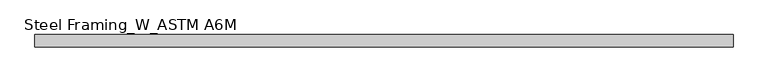
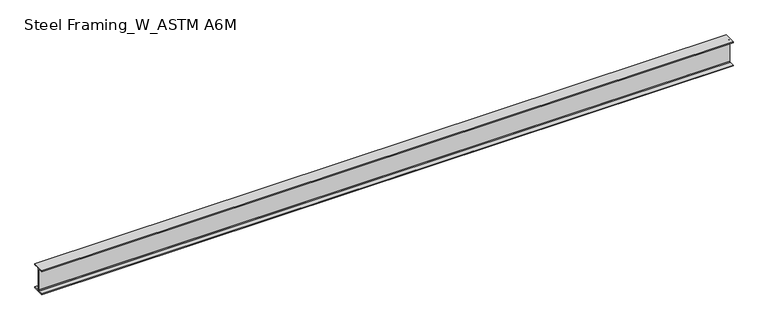
"""IFC4 building model written with IfcOpenShell, lengths in millimetres: beam geometry, Steel Framing_W_ASTM A6M : H_SB_AR_S02_W360x51_B4."""

from ifc_helpers import new_model, si_unit, point, frame, frame_2d, origin, place, context, project, spatial, polyline, circle_curve, trimmed, segment, composite_curve, outline, extrude, source, transform, mapped, element, save


def steel_framing_w_astm_a6m_bf6e2db3(model_context):
    return source(origin(), model_context, "Body", "SweptSolid", [
        extrude(outline(composite_curve([segment(polyline([(85.5, -166.4), (85.5, -178.0), (-85.5, -178.0), (-85.5, -166.4), (-13.72, -166.4)]), True, "CONTINUOUS"), segment(trimmed(circle_curve(frame_2d((-13.72, -156.3)), 10.1), [point((-13.72, -166.4))], [point((-3.62, -156.3))], True, "CARTESIAN"), True, "CONTINUOUS"), segment(polyline([(-3.62, -156.3), (-3.62, 156.3)]), True, "CONTINUOUS"), segment(trimmed(circle_curve(frame_2d((-13.72, 156.3)), 10.1), [point((-3.62, 156.3))], [point((-13.72, 166.4))], True, "CARTESIAN"), True, "CONTINUOUS"), segment(polyline([(-13.72, 166.4), (-85.5, 166.4), (-85.5, 178.0), (85.5, 178.0), (85.5, 166.4), (13.72, 166.4)]), True, "CONTINUOUS"), segment(trimmed(circle_curve(frame_2d((13.72, 156.3)), 10.1), [point((13.72, 166.4))], [point((3.62, 156.3))], True, "CARTESIAN"), True, "CONTINUOUS"), segment(polyline([(3.62, 156.3), (3.62, -156.3)]), True, "CONTINUOUS"), segment(trimmed(circle_curve(frame_2d((13.72, -156.3)), 10.1), [point((3.62, -156.3))], [point((13.72, -166.4))], True, "CARTESIAN"), True, "CONTINUOUS"), segment(polyline([(13.72, -166.4), (85.5, -166.4)]), True, "CONTINUOUS")], self_intersect=False)), frame((-4814.1, 0.0, 0.0), z_axis=(1.0, 0.0, 0.0), x_axis=(0.0, 1.0, 0.0)), (0.0, 0.0, 1.0), 9715.9),
    ])


if __name__ == "__main__":
    model = new_model("IFC4")
    model_context = context("Model", 3, world=origin())
    ifc_project = project(units=[si_unit("LENGTHUNIT", "METRE", prefix="MILLI")], contexts=[model_context])
    site = spatial("IfcSite", under=ifc_project)
    building = spatial("IfcBuilding", under=site)
    placement = place(None, origin())
    steel_framing_w_astm_a6m_shape = steel_framing_w_astm_a6m_bf6e2db3(model_context)
    element("IfcBeam", 1, ObjectType="Steel Framing_W_ASTM A6M : H_SB_AR_S02_W360x51_B4", at=placement, inside=building, context=model_context, shape_type="MappedRepresentation", body=[
        mapped(steel_framing_w_astm_a6m_shape, transform((0.0, 0.0, 0.0), x_axis=(1.0, 0.0, 0.0), y_axis=(0.0, 1.0, 0.0), z_axis=(0.0, 0.0, 1.0))),
    ])
    save(model, "model.ifc")

# Revit data of these elements
# Type "Steel Framing_W_ASTM A6M : H_SB_AR_S02_W360x51_B4"
#   Type Mark = "B4"
#   Section Name Key = "W14x34"
#   Width = 17.1 cm
#   Web Thickness = 0.724 cm
#   Web Fillet = 1.01 cm
#   Warping Constant = 287000.0 cm⁶
#   Torsional Moment of Inertia = 23.70 cm⁴
#   Section Area = 64.5 cm²
#   Plastic Modulus weak axis = 174.0 cm³
#   Plastic Modulus strong axis = 895.0 cm³
#   Perimeter = 1.36 m²/m
#   Nominal Weight = 51.00 kgf/m
#   Moment of Inertia weak axis = 970.00 cm⁴
#   Moment of Inertia strong axis = 14200.00 cm⁴
#   Height = 35.6 cm
#   Flange Thickness = 1.16 cm
#   Elastic Modulus weak axis = 113.0 cm³
#   Elastic Modulus strong axis = 796.0 cm³
#   Centroid Vertical = 17.8 cm
#   Centroid Horizontal = 8.55 cm
#   Length [instance default] = 1500 mm
#   Structural Material [instance default] = Steel, 45-345
#   Bolt Spacing = 0
#   Assembly Code = ""
# Element 1 (IfcBeam, "Steel Framing_W_ASTM A6M : H_SB_AR_S02_W360x51_B4")
#   Materials on its faces: "Steel, 45-345"
# Materials
#   "Steel, 45-345": class "Metal", colour RGB 189 187 185, transparency 0, Description = "Steel 345 MPa", Cost = 0
